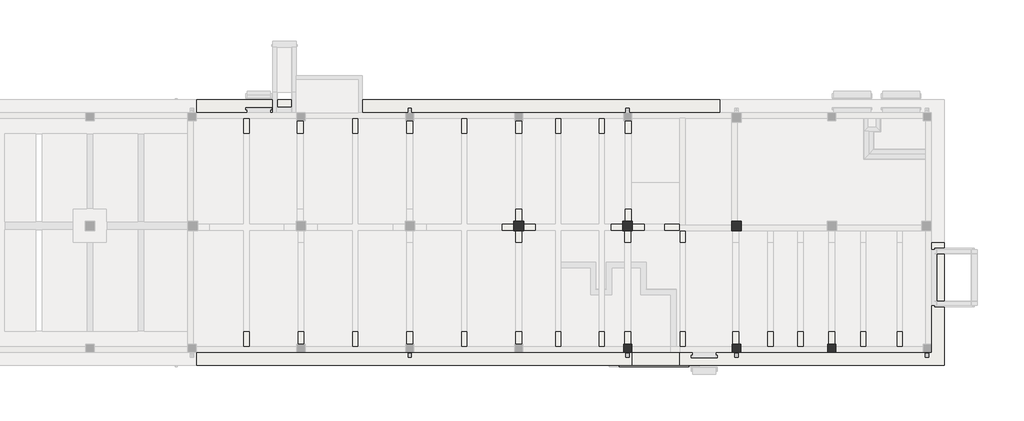
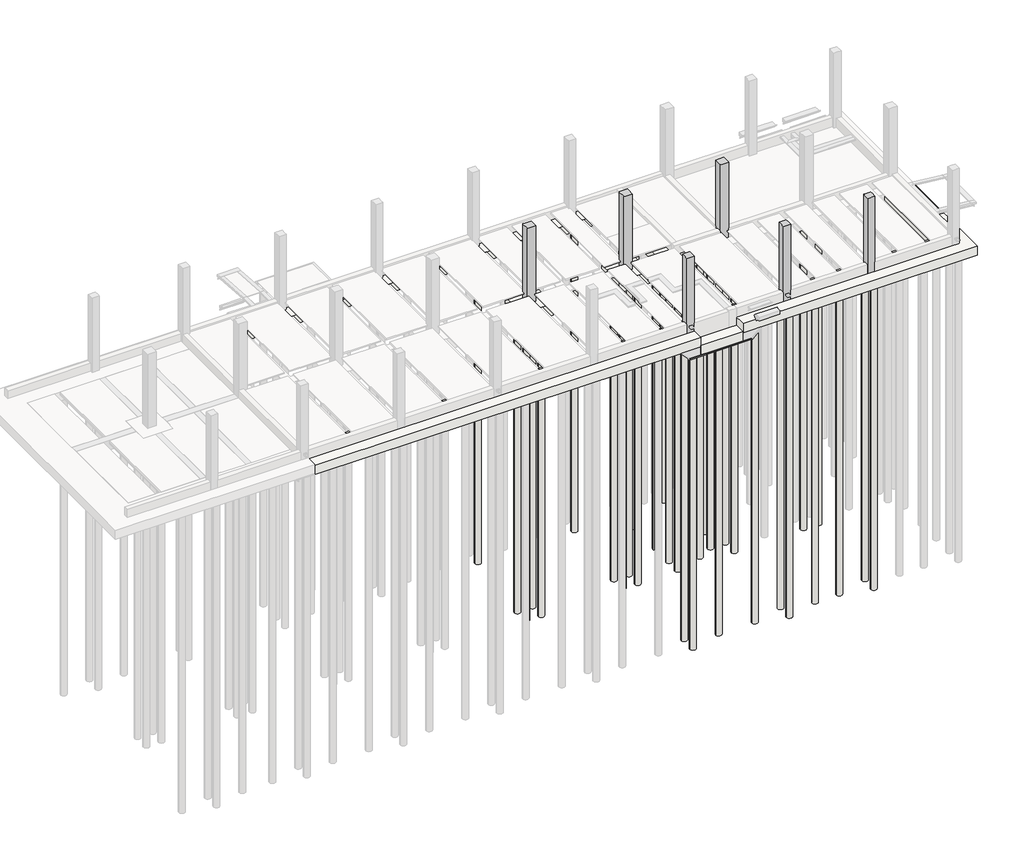
# One storey, part 5 of 7: 42 slabs, 6 columns.
"""IFC4 building model written with IfcOpenShell, lengths in millimetres."""

import ifcopenshell
import ifcopenshell.guid

model = None  # the IFC model being written
_history = None  # IfcOwnerHistory: only IFC2X3 demands one
_inside = {}  # id of a spatial element -> (the spatial element, [elements in it])
_under = {}  # id of a project, library or spatial element -> (it, [spatial elements below it])
_declared = {}  # id of a project -> (the project, [libraries it declares])
_typed = {}  # id of a type object -> (the type object, [elements of that type])
_made_of = {}  # id of a material, layer set ... -> (it, [elements and type objects made of it])


def new_model(schema):
    """Start an empty IFC model of exactly this schema.

    Asked for "IFC4X3", IfcOpenShell would pick the latest addendum, in which some entities
    have other attributes; the version numbers below select the first issue.
    IFC2X3 requires an IfcOwnerHistory on every rooted entity: one is made here for all.
    """
    global model, _history
    if schema == "IFC4X3":
        model = ifcopenshell.file(schema_version=(4, 3, 0, 0))
    else:
        model = ifcopenshell.file(schema=schema)
    _inside.clear()
    _under.clear()
    _declared.clear()
    _typed.clear()
    _made_of.clear()
    _history = None
    if model.schema == "IFC2X3":
        org = make("IfcOrganization", Name="unknown")
        user = make(
            "IfcPersonAndOrganization",
            ThePerson=make("IfcPerson", FamilyName="unknown"),
            TheOrganization=org,
        )
        app = make(
            "IfcApplication",
            ApplicationDeveloper=org,
            Version="unknown",
            ApplicationFullName="unknown",
            ApplicationIdentifier="unknown",
        )
        _history = make(
            "IfcOwnerHistory",
            OwningUser=user,
            OwningApplication=app,
            ChangeAction="ADDED",
            CreationDate=0,
        )
    return model


def make(cls, **values):
    """One entity of the class cls with the attributes given. An attribute that is None is left unset."""
    return model.create_entity(
        cls, **{name: value for name, value in values.items() if value is not None}
    )


def rooted(cls, **values):
    """An entity with a GlobalId (a new one), such as an element, a storey or a relation."""
    return make(cls, GlobalId=ifcopenshell.guid.new(), OwnerHistory=_history, **values)


def si_unit(unit_type, name, prefix=None):
    """IfcSIUnit, for example si_unit("LENGTHUNIT", "METRE", prefix="MILLI")."""
    return make("IfcSIUnit", UnitType=unit_type, Prefix=prefix, Name=name)


def assignment(units):
    """IfcUnitAssignment: the units of a project."""
    return None if units is None else make("IfcUnitAssignment", Units=units)


def point(xyz):
    """IfcCartesianPoint."""
    return None if xyz is None else make("IfcCartesianPoint", Coordinates=xyz)


def direction(xyz):
    """IfcDirection."""
    return None if xyz is None else make("IfcDirection", DirectionRatios=xyz)


def frame(location, z_axis=None, x_axis=None):
    """IfcAxis2Placement3D, a coordinate frame: its origin and axes. An axis left out is left unset."""
    return make(
        "IfcAxis2Placement3D",
        Location=point(location),
        Axis=direction(z_axis),
        RefDirection=direction(x_axis),
    )


def frame_2d(location, x_axis=None):
    """IfcAxis2Placement2D, a coordinate frame in the plane: its origin and x axis."""
    return make(
        "IfcAxis2Placement2D", Location=point(location), RefDirection=direction(x_axis)
    )


def origin():
    """The frame at (0, 0, 0) with its axes left unset."""
    return frame((0.0, 0.0, 0.0))


def place(relative_to, where):
    """IfcLocalPlacement: puts the frame where relative to a parent placement (None: the world)."""
    return make(
        "IfcLocalPlacement", PlacementRelTo=relative_to, RelativePlacement=where
    )


def context(
    kind, dimensions, precision=None, world=None, true_north=None, identifier=None
):
    """IfcGeometricRepresentationContext, for example the 3D "Model" context."""
    return make(
        "IfcGeometricRepresentationContext",
        ContextIdentifier=identifier,
        ContextType=kind,
        CoordinateSpaceDimension=dimensions,
        Precision=precision,
        WorldCoordinateSystem=world,
        TrueNorth=true_north,
    )


def project(units=None, contexts=None):
    """IfcProject with its units and contexts."""
    return rooted(
        "IfcProject",
        Name="project",
        RepresentationContexts=contexts,
        UnitsInContext=assignment(units),
    )


def spatial(cls, under=None, at=None, **own):
    """A site, building, storey or space (cls), placed at a placement, below another one or the project."""
    s = rooted(cls, ObjectPlacement=at, **own)
    if under is not None:
        _under.setdefault(under.id(), (under, []))[1].append(s)
    return s


def polyline(points):
    """IfcPolyline through the points."""
    return make("IfcPolyline", Points=[point(p) for p in points])


def circle_curve(where, radius):
    """IfcCircle in the frame where."""
    return make("IfcCircle", Position=where, Radius=radius)


def trimmed(basis, trim1, trim2, sense, master):
    """IfcTrimmedCurve: the piece of a basis curve between two trims."""
    return make(
        "IfcTrimmedCurve",
        BasisCurve=basis,
        Trim1=trim1,
        Trim2=trim2,
        SenseAgreement=sense,
        MasterRepresentation=master,
    )


def segment(curve, same_sense, transition):
    """IfcCompositeCurveSegment."""
    return make(
        "IfcCompositeCurveSegment",
        Transition=transition,
        SameSense=same_sense,
        ParentCurve=curve,
    )


def composite_curve(segments, self_intersect=None):
    """IfcCompositeCurve: segments joined end to end."""
    return make("IfcCompositeCurve", Segments=segments, SelfIntersect=self_intersect)


def outline(outer, holes=None, kind="AREA"):
    """IfcArbitraryClosedProfileDef: a profile drawn as a closed curve; with holes, ...WithVoids."""
    if holes is None:
        return make("IfcArbitraryClosedProfileDef", ProfileType=kind, OuterCurve=outer)
    return make(
        "IfcArbitraryProfileDefWithVoids",
        ProfileType=kind,
        OuterCurve=outer,
        InnerCurves=holes,
    )


def extrude(swept, where, along, depth):
    """IfcExtrudedAreaSolid: the profile swept, set in the frame where, extruded along a direction by depth."""
    return make(
        "IfcExtrudedAreaSolid",
        SweptArea=swept,
        Position=where,
        ExtrudedDirection=direction(along),
        Depth=depth,
    )


def faces_of(points, faces, orient=None, outer=None):
    """IfcFace entities. A face is a list of loops; a loop is a list of indices into points, from 0.

    orient and outer hold one flag for each loop. By default every Orientation is true, the
    first loop of a face is its IfcFaceOuterBound and the others are IfcFaceBound.
    """
    made = []
    for i, loops in enumerate(faces):
        bounds = []
        for j, loop in enumerate(loops):
            is_outer = j == 0 if outer is None else outer[i][j]
            bounds.append(
                make(
                    "IfcFaceOuterBound" if is_outer else "IfcFaceBound",
                    Bound=make("IfcPolyLoop", Polygon=[points[k] for k in loop]),
                    Orientation=True if orient is None else orient[i][j],
                )
            )
        made.append(make("IfcFace", Bounds=bounds))
    return made


def faceted_brep(points, faces, orient=None, outer=None, voids=None):
    """IfcFacetedBrep: a solid bounded by flat faces; with voids (closed shells), ...WithVoids."""
    shared = [point(p) for p in points]
    hull = make("IfcClosedShell", CfsFaces=faces_of(shared, faces, orient, outer))
    if voids is None:
        return make("IfcFacetedBrep", Outer=hull)
    return make(
        "IfcFacetedBrepWithVoids",
        Outer=hull,
        Voids=[
            make(cls, CfsFaces=faces_of(shared, fs, o, b)) for cls, fs, o, b in voids
        ],
    )


def shape(context_of_items, identifier, shape_type, items):
    """IfcShapeRepresentation: the items that make up one representation, for example the "Body"."""
    return make(
        "IfcShapeRepresentation",
        ContextOfItems=context_of_items,
        RepresentationIdentifier=identifier,
        RepresentationType=shape_type,
        Items=items,
    )


def made_of(thing, what):
    """Note that an element or type object is made of a material, layer set ...; save() writes the relation."""
    if what is not None:
        _made_of.setdefault(what.id(), (what, []))[1].append(thing)
    return thing


def element(
    cls,
    number,
    at=None,
    inside=None,
    cuts=None,
    type_object=None,
    material=None,
    context=None,
    identifier="Body",
    shape_type=None,
    held_by="IfcProductDefinitionShape",
    body=None,
    shapes=None,
    **own,
):
    """One element of the class cls, such as IfcWall. Its Tag is "e" and its number.

    at: its placement. inside: the storey or other place that contains it. cuts: it is an
    opening in that element (IfcRelVoidsElement). A single representation is given by context,
    identifier, shape_type and body (its items); several are given by shapes. held_by: the class
    of the entity that holds the representations. save() writes the other relations.
    """
    e = rooted(cls, Tag="e%d" % number, ObjectPlacement=at, **own)
    if body is not None:
        shapes = [shape(context, identifier, shape_type, body)]
    if shapes is not None:
        e.Representation = make(held_by, Representations=shapes)
    if inside is not None:
        _inside.setdefault(inside.id(), (inside, []))[1].append(e)
    if cuts is not None:
        rooted(
            "IfcRelVoidsElement", RelatingBuildingElement=cuts, RelatedOpeningElement=e
        )
    if type_object is not None:
        _typed.setdefault(type_object.id(), (type_object, []))[1].append(e)
    return made_of(e, material)


def aggregate(whole, parts):
    """IfcRelAggregates: a whole, such as a stair, and the parts it consists of."""
    return rooted("IfcRelAggregates", RelatingObject=whole, RelatedObjects=parts)


def save(model, path):
    """Write the relations noted so far, then the file.

    IfcRelAggregates (storeys below a building ...), IfcRelContainedInSpatialStructure (elements
    in a storey), IfcRelDefinesByType, IfcRelAssociatesMaterial and IfcRelDeclares: one each for
    every whole, place, type object, material and project.
    """
    for whole, parts in _under.values():
        aggregate(whole, parts)
    for where, things in _inside.values():
        rooted(
            "IfcRelContainedInSpatialStructure",
            RelatedElements=things,
            RelatingStructure=where,
        )
    for kind, things in _typed.values():
        rooted("IfcRelDefinesByType", RelatedObjects=things, RelatingType=kind)
    for what, things in _made_of.values():
        rooted("IfcRelAssociatesMaterial", RelatedObjects=things, RelatingMaterial=what)
    for by, libraries in _declared.values():
        rooted("IfcRelDeclares", RelatingContext=by, RelatedDefinitions=libraries)
    model.write(path)


model = new_model("IFC4")

# Units and contexts
model_context = context("Model", 3, world=origin())
ifc_project = project(units=[si_unit("LENGTHUNIT", "METRE", prefix="MILLI")], contexts=[model_context])

# Site, building, storey
site = spatial("IfcSite", under=ifc_project)
building = spatial("IfcBuilding", under=site)
storey = spatial("IfcBuildingStorey", under=building, Name="H.P.P", Elevation=4500.0)

# Columns
placement = place(None, origin())
element("IfcColumn", 1, ObjectType="RC_Column_Rectangular : H_SC_AR S15_RC Col-AG_700x700_C1", at=placement, inside=storey, context=model_context, shape_type="Brep", body=[
    faceted_brep([(39350.0000001, -7650.0, 4000.0), (39350.0000001, -8350.0, 4000.0), (39250.0000001, -8350.0, 4000.0), (38750.0000001, -8350.0, 4000.0), (38650.0000001, -8350.0, 4000.0), (38650.0000001, -7650.0, 4000.0), (38750.0, -7650.0, 4000.0), (39250.0, -7650.0, 4000.0), (39350.0000001, -7650.0, 4650.0), (39350.0000001, -7650.0, 4800.0), (39350.0000001, -7650.0, 10450.0), (39350.0000001, -7650.0, 10600.0), (39350.0000001, -7700.0, 10600.0), (39350.0000001, -8300.0, 10600.0), (39350.0000001, -8350.0, 10600.0), (39350.0000001, -8350.0, 10450.0), (39350.0000001, -8350.0, 4800.0), (39350.0000001, -8350.0, 4650.0), (39249.9999998, -8350.0, 10600.0), (38750.0000002, -8350.0, 10600.0), (38650.0000001, -8350.0, 10600.0), (38650.0000001, -8350.0, 10450.0), (38650.0000001, -8350.0, 4800.0), (38650.0000001, -8350.0, 4650.0), (38650.0000001, -8300.0, 10600.0), (38650.0000001, -7700.0, 10600.0), (38650.0000001, -7650.0, 10600.0), (38650.0000001, -7650.0, 10450.0), (38650.0000001, -7650.0, 4800.0), (38650.0000001, -7650.0, 4650.0), (38750.0000002, -7650.0, 10600.0), (39249.9999998, -7650.0, 10600.0)], [[[0, 1, 2, 3, 4, 5, 6, 7]], [[1, 0, 8, 9, 10, 11, 12, 13, 14, 15, 16, 17]], [[4, 3, 2, 1, 17, 16, 15, 14, 18, 19, 20, 21, 22, 23]], [[5, 4, 23, 22, 21, 20, 24, 25, 26, 27, 28, 29]], [[0, 7, 6, 5, 29, 28, 27, 26, 30, 31, 11, 10, 9, 8]], [[12, 11, 31, 30, 26, 25, 24, 20, 19, 18, 14, 13]]]),
])
element("IfcColumn", 2, ObjectType="RC_Column_Rectangular : H_SC_AR S15_RC Col-AG_700x700_C1", at=placement, inside=storey, context=model_context, shape_type="Brep", body=[
    faceted_brep([(47349.9999999, -7650.0, 4000.0), (47349.9999999, -8350.0, 4000.0), (47249.9999999, -8350.0, 4000.0), (46749.9999999, -8350.0, 4000.0), (46649.9999999, -8350.0, 4000.0), (46649.9999999, -7650.0, 4000.0), (46800.0, -7650.0, 4000.0), (47300.0, -7650.0, 4000.0), (47349.9999999, -7650.0, 4650.0), (47349.9999999, -7850.0, 4650.0), (47349.9999999, -7850.0, 4800.0), (47349.9999999, -7650.0, 4800.0), (47349.9999999, -7650.0, 10450.0), (47349.9999999, -7650.0, 10600.0), (47349.9999999, -7750.0, 10600.0), (47349.9999999, -8350.0, 10600.0), (47349.9999999, -8350.0, 10450.0), (47349.9999999, -8350.0, 4800.0), (47349.9999999, -8350.0, 4650.0), (47300.0, -8350.0, 10600.0), (46800.0, -8350.0, 10600.0), (46649.9999999, -8350.0, 10600.0), (46649.9999999, -8350.0, 10450.0), (46649.9999999, -8350.0, 4800.0), (46649.9999999, -8350.0, 4650.0), (46649.9999999, -8300.0, 10600.0), (46649.9999999, -7700.0, 10600.0), (46649.9999999, -7650.0, 10600.0), (46649.9999999, -7650.0, 10450.0), (46649.9999999, -7650.0, 4800.0), (46649.9999999, -7650.0, 4650.0), (46800.0, -7650.0, 10600.0), (47300.0, -7650.0, 10600.0), (47300.0, -7650.0, 4800.0), (47300.0, -7650.0, 4650.0), (47300.0, -7850.0, 4650.0), (47300.0, -7850.0, 4800.0)], [[[0, 1, 2, 3, 4, 5, 6, 7]], [[1, 0, 8, 9, 10, 11, 12, 13, 14, 15, 16, 17, 18]], [[4, 3, 2, 1, 18, 17, 16, 15, 19, 20, 21, 22, 23, 24]], [[5, 4, 24, 23, 22, 21, 25, 26, 27, 28, 29, 30]], [[0, 7, 6, 5, 30, 29, 28, 27, 31, 32, 13, 12, 11, 33, 34, 8]], [[14, 13, 32, 31, 27, 26, 25, 21, 20, 19, 15]], [[35, 9, 8, 34]], [[10, 36, 33, 11]], [[35, 36, 10, 9]], [[36, 35, 34, 33]]]),
])
element("IfcColumn", 3, ObjectType="RC_Column_Rectangular : H_SC_AR S15_RC Col-AG_700x700_C1", at=placement, inside=storey, context=model_context, shape_type="Brep", body=[
    faceted_brep([(55350.0, -7650.0, 4000.0), (55350.0, -7950.0, 4000.0), (55350.0, -8350.0, 4000.0), (54650.0, -8350.0, 4000.0), (54650.0, -7950.0, 4000.0), (54650.0, -7650.0, 4000.0), (55050.0, -7650.0, 4000.0), (55350.0, -7650.0, 10600.0), (55350.0, -8350.0, 10600.0), (55350.0, -8350.0, 10450.0), (55350.0, -8350.0, 9800.0), (55350.0, -8350.0, 4800.0), (55350.0, -8350.0, 4650.0), (55200.0, -8350.0, 10600.0), (54700.0, -8350.0, 10600.0), (54650.0, -8350.0, 10600.0), (54650.0, -8350.0, 10450.0), (54650.0, -8350.0, 9700.0), (54650.0, -8350.0, 4800.0), (54650.0, -8350.0, 4650.0), (54650.0, -7650.0, 10600.0), (54650.0, -7650.0, 9800.0), (54650.0, -7650.0, 4800.0)], [[[0, 1, 2, 3, 4, 5, 6]], [[2, 1, 0, 7, 8, 9, 10, 11, 12]], [[3, 2, 12, 11, 10, 9, 8, 13, 14, 15, 16, 17, 18, 19]], [[5, 4, 3, 19, 18, 17, 16, 15, 20, 21, 22]], [[0, 6, 5, 22, 21, 20, 7]], [[8, 7, 20, 15, 14, 13]]]),
])
element("IfcColumn", 4, ObjectType="RC_Column_Rectangular : H_SC_AR S15_RC Col-AG_600x600_C2", at=placement, inside=storey, context=model_context, shape_type="Brep", body=[
    faceted_brep([(62300.0, -16700.0, 4000.0), (62300.0, -16900.0, 4000.0), (62300.0, -17300.0, 4000.0), (61700.0, -17300.0, 4000.0), (61700.0, -16900.0, 4000.0), (61700.0, -16700.0, 4000.0), (62300.0, -16700.0, 4650.0), (62300.0, -16700.0, 4800.0), (62300.0, -16700.0, 10450.0), (62300.0, -16700.0, 10600.0), (62300.0, -16900.0, 10600.0), (62300.0, -17300.0, 10600.0), (62300.0, -17300.0, 9800.0), (62300.0, -17300.0, 4800.0), (61700.0, -17300.0, 10600.0), (61700.0, -17300.0, 9800.0), (61700.0, -17300.0, 4800.0), (61700.0, -16900.0, 10600.0), (61700.0, -16700.0, 10600.0), (61700.0, -16700.0, 10450.0), (61700.0, -16700.0, 4800.0), (61700.0, -16700.0, 4650.0), (61750.0, -16700.0, 10600.0), (62250.0, -16700.0, 10600.0)], [[[0, 1, 2, 3, 4, 5]], [[2, 1, 0, 6, 7, 8, 9, 10, 11, 12, 13]], [[3, 2, 13, 12, 11, 14, 15, 16]], [[5, 4, 3, 16, 15, 14, 17, 18, 19, 20, 21]], [[0, 5, 21, 20, 19, 18, 22, 23, 9, 8, 7, 6]], [[14, 11, 10, 9, 23, 22, 18, 17]]]),
])
element("IfcColumn", 5, ObjectType="RC_Column_Rectangular : H_SC_AR S15_RC Col-AG_600x600_C2", at=placement, inside=storey, context=model_context, shape_type="Brep", body=[
    faceted_brep([(55300.0, -16700.0, 4000.0), (55300.0, -16900.0, 4000.0), (55300.0, -17300.0, 4000.0), (54700.0, -17300.0, 4000.0), (54700.0, -16900.0, 4000.0), (54700.0, -16700.0, 4000.0), (55300.0, -16700.0, 4650.0), (55300.0, -16700.0, 4800.0), (55300.0, -16700.0, 10450.0), (55300.0, -16700.0, 10600.0), (55300.0, -16900.0, 10600.0), (55300.0, -17300.0, 10600.0), (55300.0, -17300.0, 9800.0), (55300.0, -17300.0, 4800.0), (54700.0, -17300.0, 10600.0), (54700.0, -17300.0, 9800.0), (54700.0, -17300.0, 4800.0), (54700.0, -16900.0, 10600.0), (54700.0, -16700.0, 10600.0), (54700.0, -16700.0, 10450.0), (54700.0, -16700.0, 9800.0), (54700.0, -16700.0, 4800.0), (54700.0, -16700.0, 4650.0), (55200.0, -16700.0, 10600.0)], [[[0, 1, 2, 3, 4, 5]], [[2, 1, 0, 6, 7, 8, 9, 10, 11, 12, 13]], [[3, 2, 13, 12, 11, 14, 15, 16]], [[5, 4, 3, 16, 15, 14, 17, 18, 19, 20, 21, 22]], [[0, 5, 22, 21, 20, 19, 18, 23, 9, 8, 7, 6]], [[14, 11, 10, 9, 23, 18, 17]]]),
])
element("IfcColumn", 6, ObjectType="RC_Column_Rectangular : H_SC_AR S15_RC Col-AG_600x600_C2", at=placement, inside=storey, context=model_context, shape_type="Brep", body=[
    faceted_brep([(46700.0, -16700.0, 4000.0), (47300.0, -16700.0, 4000.0), (47300.0, -17300.0, 4000.0), (46700.0, -17300.0, 4000.0), (46700.0, -16900.0, 4000.0), (46700.0, -16700.0, 4550.0), (46700.0, -16700.0, 4700.0), (46700.0, -16700.0, 10450.0), (46700.0, -16700.0, 10600.0), (46800.0, -16700.0, 10600.0), (47300.0, -16700.0, 10600.0), (47300.0, -16700.0, 10450.0), (47300.0, -16700.0, 4700.0), (47300.0, -16700.0, 4550.0), (47300.0, -16900.0, 10600.0), (47300.0, -17300.0, 10600.0), (47300.0, -17300.0, 9800.0), (47300.0, -17300.0, 4700.0), (46700.0, -17300.0, 10600.0), (46700.0, -17300.0, 9800.0), (46700.0, -17300.0, 4800.0), (46700.0, -16900.0, 10600.0)], [[[0, 1, 2, 3, 4]], [[1, 0, 5, 6, 7, 8, 9, 10, 11, 12, 13]], [[2, 1, 13, 12, 11, 10, 14, 15, 16, 17]], [[3, 2, 17, 16, 15, 18, 19, 20]], [[0, 4, 3, 20, 19, 18, 21, 8, 7, 6, 5]], [[18, 15, 14, 10, 9, 8, 21]]]),
])

# Slabs
element("IfcSlab", 7, ObjectType="H_SF_AR S18_MAT_T800_WF1", at=placement, inside=storey, context=model_context, shape_type="Brep", body=[
    faceted_brep([(50825.0, -18250.0000001, 3200.0), (50825.0, -15750.0000001, 3200.0), (52225.0, -15750.0000001, 3200.0), (67750.0000002, -15750.0000001, 3200.0), (67750.0000002, -9250.0, 3200.0), (70250.0, -9250.0, 3200.0), (70250.0, -18250.0000001, 3200.0), (52225.0, -18250.0000001, 3200.0), (50825.0, -18250.0000001, 4000.0), (70250.0, -18250.0000001, 4000.0), (70250.0, -9250.0, 4000.0), (67750.0000002, -9250.0, 4000.0), (67750.0000002, -15750.0000001, 4000.0), (50825.0, -15750.0000001, 4000.0), (50825.0, -16900.0, 4000.0), (50825.0, -18250.0000001, 3300.0), (50825.0, -15750.0000001, 3300.0)], [[[0, 1, 2, 3, 4, 5, 6, 7]], [[8, 9, 10, 11, 12, 13, 14]], [[6, 5, 10, 9]], [[0, 7, 6, 9, 8, 15]], [[3, 2, 1, 16, 13, 12]], [[4, 3, 12, 11]], [[1, 0, 15, 8, 14, 13, 16]], [[5, 4, 11, 10]]]),
    faceted_brep([(15299.9999999, -18250.0000001, 3200.0), (15299.9999999, -15750.0000001, 3200.0), (45675.0, -15750.0000001, 3200.0), (47300.0, -15750.0000001, 3200.0), (47300.0, -18250.0000001, 3200.0), (45675.0, -18250.0000001, 3200.0), (15299.9999999, -18250.0000001, 4000.0), (47300.0, -18250.0000001, 4000.0), (47300.0, -15750.0000001, 4000.0), (15299.9999999, -15750.0000001, 4000.0), (15299.9999999, -18250.0000001, 3300.0), (15299.9999999, -15750.0000001, 3300.0), (47300.0, -15750.0000001, 3300.0), (47300.0, -18250.0000001, 3300.0)], [[[0, 1, 2, 3, 4, 5]], [[6, 7, 8, 9]], [[1, 0, 10, 6, 9, 11]], [[3, 2, 1, 11, 9, 8, 12]], [[4, 3, 12, 8, 7, 13]], [[0, 5, 4, 13, 7, 6, 10]]]),
    faceted_brep([(53749.9998007, 1249.9999999, 3200.0), (53749.9998007, -1250.0000001, 3200.0), (52200.0000002, -1250.0000001, 3200.0), (52200.0000002, -6750.0000001, 3200.0), (53749.9998007, -6750.0000001, 3200.0), (53749.9998007, -9250.0, 3200.0), (49700.0000002, -9250.0, 3200.0), (49700.0000002, -1250.0000001, 3200.0), (15299.9999999, -1250.0000001, 3200.0), (15299.9999999, 1249.9999999, 3200.0), (53749.9998007, 1249.9999999, 4000.0), (15299.9999999, 1249.9999999, 4000.0), (15299.9999999, -1250.0000001, 4000.0), (49700.0000002, -1250.0000001, 4000.0), (49700.0000002, -9250.0, 4000.0), (53749.9998007, -9250.0, 4000.0), (53749.9998007, -6750.0000001, 4000.0), (52200.0000002, -6750.0000001, 4000.0), (52200.0000002, -1250.0000001, 4000.0), (53749.9998007, -1250.0000001, 4000.0), (15299.9999999, 1249.9999999, 3300.0), (15299.9999999, -1250.0000001, 3300.0)], [[[0, 1, 2, 3, 4, 5, 6, 7, 8, 9]], [[10, 11, 12, 13, 14, 15, 16, 17, 18, 19]], [[0, 9, 20, 11, 10]], [[6, 5, 15, 14]], [[7, 6, 14, 13]], [[8, 7, 13, 12, 21]], [[2, 1, 19, 18]], [[3, 2, 18, 17]], [[4, 3, 17, 16]], [[1, 0, 10, 19]], [[9, 8, 21, 12, 11, 20]], [[5, 4, 16, 15]]]),
])
element("IfcSlab", 8, ObjectType="H_SF_AR S18_MAT_T800_WF1", at=placement, inside=storey, context=model_context, shape_type="Brep", body=[
    faceted_brep([(50825.0, -15750.0000001, 2500.0), (50825.0, -18250.0000001, 2500.0), (47300.0, -18250.0000001, 2500.0), (47300.0, -15750.0000001, 2500.0), (50825.0, -18250.0000001, 3300.0), (50825.0, -15750.0000001, 3300.0), (47300.0, -15750.0000001, 3300.0), (47300.0, -18250.0000001, 3300.0), (50825.0, -15750.0000001, 3200.0), (50825.0, -18250.0000001, 3200.0), (47300.0, -18250.0000001, 3200.0), (47300.0, -15750.0000001, 3200.0)], [[[0, 1, 2, 3]], [[4, 5, 6, 7]], [[1, 0, 8, 5, 4, 9]], [[2, 1, 9, 4, 7, 10]], [[3, 2, 10, 7, 6, 11]], [[0, 3, 11, 6, 5, 8]]]),
])
element("IfcSlab", 9, ObjectType="H_SF_AR_S18_Lean_T50", at=placement, inside=storey, context=model_context, shape_type="SweptSolid", body=[
    extrude(outline(polyline([(51525.0, -15650.0), (51525.0, -18350.0000001), (46375.0, -18350.0000001), (46375.0, -15650.0), (51525.0, -15650.0)])), frame((0.0, 0.0, 2450.0), z_axis=(0.0, 0.0, 1.0), x_axis=(1.0, 0.0, 0.0)), (0.0, 0.0, 1.0), 50.0),
])
element("IfcSlab", 10, ObjectType="H_SF_AR_S18_Lean_T50", at=placement, inside=storey, context=model_context, shape_type="Brep", body=[
    faceted_brep([(50475.0, -16790.0, 4390.0), (47360.0, -16790.0, 4390.0), (47360.0, -10775.0, 4390.0), (48275.0, -10775.0, 4390.0), (48275.0, -12775.0, 4390.0), (50475.0, -12775.0, 4390.0), (47360.0, -16790.0, 4440.0), (50475.0, -16790.0, 4440.0), (50475.0, -12775.0, 4440.0), (48275.0, -12775.0, 4440.0), (48275.0, -10775.0, 4440.0), (47360.0, -10775.0, 4440.0)], [[[0, 1, 2, 3, 4, 5]], [[6, 7, 8, 9, 10, 11]], [[1, 0, 7, 6]], [[2, 1, 6, 11]], [[3, 2, 11, 10]], [[4, 3, 10, 9]], [[5, 4, 9, 8]], [[0, 5, 8, 7]]]),
    faceted_brep([(46640.0, -10775.0, 4390.0), (46640.0, -16790.0, 4390.0), (45435.0, -16790.0, 4390.0), (45435.0, -12775.0, 4390.0), (45504.2893219, -12775.0, 4390.0), (45525.0, -12775.0, 4390.0), (45525.0, -10775.0, 4390.0), (46640.0, -16790.0, 4440.0), (46640.0, -10775.0, 4440.0), (45525.0, -10775.0, 4440.0), (45525.0, -12775.0, 4440.0), (45454.2893219, -12775.0, 4440.0), (45435.0, -12775.0, 4440.0), (45435.0, -16790.0, 4440.0)], [[[0, 1, 2, 3, 4, 5, 6]], [[7, 8, 9, 10, 11, 12, 13]], [[1, 0, 8, 7]], [[2, 1, 7, 13]], [[3, 2, 13, 12]], [[3, 12, 11, 10, 5, 4]], [[6, 5, 10, 9]], [[0, 6, 9, 8]]]),
    faceted_brep([(44765.0, -12775.0, 4390.0), (44765.0, -16790.0, 4390.0), (42235.0, -16790.0, 4390.0), (42235.0, -10775.0, 4390.0), (44575.0, -10775.0, 4390.0), (44575.0, -12775.0, 4390.0), (44765.0, -16790.0, 4440.0), (44765.0, -12775.0, 4440.0), (44575.0, -12775.0, 4440.0), (44575.0, -10775.0, 4440.0), (42235.0, -10775.0, 4440.0), (42235.0, -16790.0, 4440.0)], [[[0, 1, 2, 3, 4, 5]], [[6, 7, 8, 9, 10, 11]], [[1, 0, 7, 6]], [[2, 1, 6, 11]], [[3, 2, 11, 10]], [[4, 3, 10, 9]], [[5, 4, 9, 8]], [[0, 5, 8, 7]]]),
    faceted_brep([(47410.0, -4825.0, 4390.0), (47410.0, -210.0, 4390.0), (50825.0, -210.0, 4390.0), (50825.0, -4825.0, 4390.0), (47410.0, -210.0, 4440.0), (47410.0, -4825.0, 4440.0), (50825.0, -4825.0, 4440.0), (50825.0, -210.0, 4440.0)], [[[0, 1, 2, 3]], [[4, 5, 6, 7]], [[1, 0, 5, 4]], [[2, 1, 4, 7]], [[3, 2, 7, 6]], [[0, 3, 6, 5]]]),
])
element("IfcSlab", 11, ObjectType="H_SF_AR_S18_Lean_T50", at=placement, inside=storey, context=model_context, shape_type="SweptSolid", body=[
    extrude(outline(polyline([(54650.0, -100.0), (54650.0, -7950.0), (51225.0, -7950.0), (51225.0, -100.0), (54650.0, -100.0)])), frame((0.0, 0.0, 4440.0), z_axis=(0.0, 0.0, 1.0), x_axis=(1.0, 0.0, 0.0)), (0.0, 0.0, 1.0), 50.0),
])
element("IfcSlab", 12, ObjectType="Foundation Rectangular (Non-Pile) : H_SF_AR S18_Ret Fdn_2500x2500xT1000_F1A", at=placement, inside=storey, context=model_context, shape_type="SweptSolid", body=[
    extrude(outline(polyline([(40250.0000001, -6750.0), (40250.0000001, -9250.0), (37750.0000001, -9250.0), (37750.0000001, -6750.0), (40250.0000001, -6750.0)])), frame((0.0, 0.0, 3000.0), z_axis=(0.0, 0.0, 1.0), x_axis=(1.0, 0.0, 0.0)), (0.0, 0.0, 1.0), 1000.0),
])
element("IfcSlab", 13, ObjectType="Foundation Rectangular (Non-Pile) : H_SF_AR S18_Ret Fdn_2500x2500xT1000_F1A", at=placement, inside=storey, context=model_context, shape_type="SweptSolid", body=[
    extrude(outline(polyline([(48249.9999999, -6750.0), (48249.9999999, -9250.0), (45749.9999999, -9250.0), (45749.9999999, -6750.0), (48249.9999999, -6750.0)])), frame((0.0, 0.0, 3000.0), z_axis=(0.0, 0.0, 1.0), x_axis=(1.0, 0.0, 0.0)), (0.0, 0.0, 1.0), 1000.0),
])
element("IfcSlab", 14, ObjectType="PILE : H_FL_AR S19_Pile_D500_L26.8", at=placement, inside=storey, context=model_context, shape_type="SweptSolid", body=[
    extrude(outline(composite_curve([segment(trimmed(circle_curve(frame_2d((39000.0, -625.0)), 250.0), [point((38750.0, -625.0))], [point((39250.0, -625.0))], False, "CARTESIAN"), True, "CONTINUOUS"), segment(trimmed(circle_curve(frame_2d((39000.0, -625.0)), 250.0), [point((39250.0, -625.0))], [point((38750.0, -625.0))], False, "CARTESIAN"), True, "CONTINUOUS")], self_intersect=False)), frame((0.0, 0.0, -23500.0), z_axis=(0.0, 0.0, 1.0), x_axis=(1.0, 0.0, 0.0)), (0.0, 0.0, 1.0), 26650.0),
])
element("IfcSlab", 15, ObjectType="PILE : H_FL_AR S19_Pile_D500_L26.8", at=placement, inside=storey, context=model_context, shape_type="SweptSolid", body=[
    extrude(outline(composite_curve([segment(trimmed(circle_curve(frame_2d((47000.0, -625.0000002)), 250.0), [point((46750.0, -625.0000002))], [point((47250.0, -625.0000002))], False, "CARTESIAN"), True, "CONTINUOUS"), segment(trimmed(circle_curve(frame_2d((47000.0, -625.0000002)), 250.0), [point((47250.0, -625.0000002))], [point((46750.0, -625.0000002))], False, "CARTESIAN"), True, "CONTINUOUS")], self_intersect=False)), frame((0.0, 0.0, -23500.0), z_axis=(0.0, 0.0, 1.0), x_axis=(1.0, 0.0, 0.0)), (0.0, 0.0, 1.0), 26650.0),
])
element("IfcSlab", 16, ObjectType="PILE : H_FL_AR S19_Pile_D500_L26.8", at=placement, inside=storey, context=model_context, shape_type="SweptSolid", body=[
    extrude(outline(composite_curve([segment(trimmed(circle_curve(frame_2d((50950.0000002, -625.0)), 250.0), [point((50700.0000002, -625.0))], [point((51200.0000002, -625.0))], False, "CARTESIAN"), True, "CONTINUOUS"), segment(trimmed(circle_curve(frame_2d((50950.0000002, -625.0)), 250.0), [point((51200.0000002, -625.0))], [point((50700.0000002, -625.0))], False, "CARTESIAN"), True, "CONTINUOUS")], self_intersect=False)), frame((0.0, 0.0, -23500.0), z_axis=(0.0, 0.0, 1.0), x_axis=(1.0, 0.0, 0.0)), (0.0, 0.0, 1.0), 26650.0),
])
element("IfcSlab", 17, ObjectType="PILE : H_FL_AR S19_Pile_D500_L26.8", at=placement, inside=storey, context=model_context, shape_type="SweptSolid", body=[
    extrude(outline(composite_curve([segment(trimmed(circle_curve(frame_2d((50950.0000002, -2500.0)), 250.0), [point((50700.0000002, -2500.0))], [point((51200.0000002, -2500.0))], False, "CARTESIAN"), True, "CONTINUOUS"), segment(trimmed(circle_curve(frame_2d((50950.0000002, -2500.0)), 250.0), [point((51200.0000002, -2500.0))], [point((50700.0000002, -2500.0))], False, "CARTESIAN"), True, "CONTINUOUS")], self_intersect=False)), frame((0.0, 0.0, -23500.0), z_axis=(0.0, 0.0, 1.0), x_axis=(1.0, 0.0, 0.0)), (0.0, 0.0, 1.0), 26650.0),
])
element("IfcSlab", 18, ObjectType="PILE : H_FL_AR S19_Pile_D500_L26.8", at=placement, inside=storey, context=model_context, shape_type="SweptSolid", body=[
    extrude(outline(composite_curve([segment(trimmed(circle_curve(frame_2d((50950.0000002, -5500.0)), 250.0), [point((50700.0000002, -5500.0))], [point((51200.0000002, -5500.0))], False, "CARTESIAN"), True, "CONTINUOUS"), segment(trimmed(circle_curve(frame_2d((50950.0000002, -5500.0)), 250.0), [point((51200.0000002, -5500.0))], [point((50700.0000002, -5500.0))], False, "CARTESIAN"), True, "CONTINUOUS")], self_intersect=False)), frame((0.0, 0.0, -23500.0), z_axis=(0.0, 0.0, 1.0), x_axis=(1.0, 0.0, 0.0)), (0.0, 0.0, 1.0), 26650.0),
])
element("IfcSlab", 19, ObjectType="PILE : H_FL_AR S19_Pile_D500_L26.8", at=placement, inside=storey, context=model_context, shape_type="SweptSolid", body=[
    extrude(outline(composite_curve([segment(trimmed(circle_curve(frame_2d((50950.0000002, -7375.0000222)), 250.0), [point((50700.0000002, -7375.0000222))], [point((51200.0000002, -7375.0000222))], False, "CARTESIAN"), True, "CONTINUOUS"), segment(trimmed(circle_curve(frame_2d((50950.0000002, -7375.0000222)), 250.0), [point((51200.0000002, -7375.0000222))], [point((50700.0000002, -7375.0000222))], False, "CARTESIAN"), True, "CONTINUOUS")], self_intersect=False)), frame((0.0, 0.0, -23500.0), z_axis=(0.0, 0.0, 1.0), x_axis=(1.0, 0.0, 0.0)), (0.0, 0.0, 1.0), 26650.0),
])
element("IfcSlab", 20, ObjectType="PILE : H_FL_AR S19_Pile_D500_L26.8", at=placement, inside=storey, context=model_context, shape_type="SweptSolid", body=[
    extrude(outline(composite_curve([segment(trimmed(circle_curve(frame_2d((50950.0000002, -8625.0000222)), 250.0), [point((50700.0000002, -8625.0000222))], [point((51200.0000002, -8625.0000222))], False, "CARTESIAN"), True, "CONTINUOUS"), segment(trimmed(circle_curve(frame_2d((50950.0000002, -8625.0000222)), 250.0), [point((51200.0000002, -8625.0000222))], [point((50700.0000002, -8625.0000222))], False, "CARTESIAN"), True, "CONTINUOUS")], self_intersect=False)), frame((0.0, 0.0, -23500.0), z_axis=(0.0, 0.0, 1.0), x_axis=(1.0, 0.0, 0.0)), (0.0, 0.0, 1.0), 26650.0),
])
element("IfcSlab", 21, ObjectType="PILE : H_FL_AR S19_Pile_D500_L26.8", at=placement, inside=storey, context=model_context, shape_type="SweptSolid", body=[
    extrude(outline(composite_curve([segment(trimmed(circle_curve(frame_2d((53125.0, -8000.0)), 250.0), [point((52875.0, -8000.0))], [point((53375.0, -8000.0))], False, "CARTESIAN"), True, "CONTINUOUS"), segment(trimmed(circle_curve(frame_2d((53125.0, -8000.0)), 250.0), [point((53375.0, -8000.0))], [point((52875.0, -8000.0))], False, "CARTESIAN"), True, "CONTINUOUS")], self_intersect=False)), frame((0.0, 0.0, -23500.0), z_axis=(0.0, 0.0, 1.0), x_axis=(1.0, 0.0, 0.0)), (0.0, 0.0, 1.0), 26650.0),
])
element("IfcSlab", 22, ObjectType="PILE : H_FL_AR S19_Pile_D500_L26.6", at=placement, inside=storey, context=model_context, shape_type="SweptSolid", body=[
    extrude(outline(composite_curve([segment(trimmed(circle_curve(frame_2d((38375.0000004, -7374.9999999)), 250.0), [point((38125.0000004, -7374.9999999))], [point((38625.0000004, -7374.9999999))], False, "CARTESIAN"), True, "CONTINUOUS"), segment(trimmed(circle_curve(frame_2d((38375.0000004, -7374.9999999)), 250.0), [point((38625.0000004, -7374.9999999))], [point((38125.0000004, -7374.9999999))], False, "CARTESIAN"), True, "CONTINUOUS")], self_intersect=False)), frame((0.0, 0.0, -23500.0), z_axis=(0.0, 0.0, 1.0), x_axis=(1.0, 0.0, 0.0)), (0.0, 0.0, 1.0), 26450.0),
])
element("IfcSlab", 23, ObjectType="PILE : H_FL_AR S19_Pile_D500_L26.6", at=placement, inside=storey, context=model_context, shape_type="SweptSolid", body=[
    extrude(outline(composite_curve([segment(trimmed(circle_curve(frame_2d((39625.0000004, -7374.9999999)), 250.0), [point((39375.0000004, -7374.9999999))], [point((39875.0000004, -7374.9999999))], False, "CARTESIAN"), True, "CONTINUOUS"), segment(trimmed(circle_curve(frame_2d((39625.0000004, -7374.9999999)), 250.0), [point((39875.0000004, -7374.9999999))], [point((39375.0000004, -7374.9999999))], False, "CARTESIAN"), True, "CONTINUOUS")], self_intersect=False)), frame((0.0, 0.0, -23500.0), z_axis=(0.0, 0.0, 1.0), x_axis=(1.0, 0.0, 0.0)), (0.0, 0.0, 1.0), 26450.0),
])
element("IfcSlab", 24, ObjectType="PILE : H_FL_AR S19_Pile_D500_L26.6", at=placement, inside=storey, context=model_context, shape_type="SweptSolid", body=[
    extrude(outline(composite_curve([segment(trimmed(circle_curve(frame_2d((38375.0000004, -8624.9999999)), 250.0), [point((38125.0000004, -8624.9999999))], [point((38625.0000004, -8624.9999999))], False, "CARTESIAN"), True, "CONTINUOUS"), segment(trimmed(circle_curve(frame_2d((38375.0000004, -8624.9999999)), 250.0), [point((38625.0000004, -8624.9999999))], [point((38125.0000004, -8624.9999999))], False, "CARTESIAN"), True, "CONTINUOUS")], self_intersect=False)), frame((0.0, 0.0, -23500.0), z_axis=(0.0, 0.0, 1.0), x_axis=(1.0, 0.0, 0.0)), (0.0, 0.0, 1.0), 26450.0),
])
element("IfcSlab", 25, ObjectType="PILE : H_FL_AR S19_Pile_D500_L26.6", at=placement, inside=storey, context=model_context, shape_type="SweptSolid", body=[
    extrude(outline(composite_curve([segment(trimmed(circle_curve(frame_2d((39625.0000004, -8624.9999999)), 250.0), [point((39375.0000004, -8624.9999999))], [point((39875.0000004, -8624.9999999))], False, "CARTESIAN"), True, "CONTINUOUS"), segment(trimmed(circle_curve(frame_2d((39625.0000004, -8624.9999999)), 250.0), [point((39875.0000004, -8624.9999999))], [point((39375.0000004, -8624.9999999))], False, "CARTESIAN"), True, "CONTINUOUS")], self_intersect=False)), frame((0.0, 0.0, -23500.0), z_axis=(0.0, 0.0, 1.0), x_axis=(1.0, 0.0, 0.0)), (0.0, 0.0, 1.0), 26450.0),
])
element("IfcSlab", 26, ObjectType="PILE : H_FL_AR S19_Pile_D500_L26.6", at=placement, inside=storey, context=model_context, shape_type="SweptSolid", body=[
    extrude(outline(composite_curve([segment(trimmed(circle_curve(frame_2d((46375.0000004, -7374.9999999)), 250.0), [point((46125.0000004, -7374.9999999))], [point((46625.0000004, -7374.9999999))], False, "CARTESIAN"), True, "CONTINUOUS"), segment(trimmed(circle_curve(frame_2d((46375.0000004, -7374.9999999)), 250.0), [point((46625.0000004, -7374.9999999))], [point((46125.0000004, -7374.9999999))], False, "CARTESIAN"), True, "CONTINUOUS")], self_intersect=False)), frame((0.0, 0.0, -23500.0), z_axis=(0.0, 0.0, 1.0), x_axis=(1.0, 0.0, 0.0)), (0.0, 0.0, 1.0), 26450.0),
])
element("IfcSlab", 27, ObjectType="PILE : H_FL_AR S19_Pile_D500_L26.6", at=placement, inside=storey, context=model_context, shape_type="SweptSolid", body=[
    extrude(outline(composite_curve([segment(trimmed(circle_curve(frame_2d((47625.0000004, -7374.9999999)), 250.0), [point((47375.0000004, -7374.9999999))], [point((47875.0000004, -7374.9999999))], False, "CARTESIAN"), True, "CONTINUOUS"), segment(trimmed(circle_curve(frame_2d((47625.0000004, -7374.9999999)), 250.0), [point((47875.0000004, -7374.9999999))], [point((47375.0000004, -7374.9999999))], False, "CARTESIAN"), True, "CONTINUOUS")], self_intersect=False)), frame((0.0, 0.0, -23500.0), z_axis=(0.0, 0.0, 1.0), x_axis=(1.0, 0.0, 0.0)), (0.0, 0.0, 1.0), 26450.0),
])
element("IfcSlab", 28, ObjectType="PILE : H_FL_AR S19_Pile_D500_L26.6", at=placement, inside=storey, context=model_context, shape_type="SweptSolid", body=[
    extrude(outline(composite_curve([segment(trimmed(circle_curve(frame_2d((46375.0000004, -8624.9999999)), 250.0), [point((46125.0000004, -8624.9999999))], [point((46625.0000004, -8624.9999999))], False, "CARTESIAN"), True, "CONTINUOUS"), segment(trimmed(circle_curve(frame_2d((46375.0000004, -8624.9999999)), 250.0), [point((46625.0000004, -8624.9999999))], [point((46125.0000004, -8624.9999999))], False, "CARTESIAN"), True, "CONTINUOUS")], self_intersect=False)), frame((0.0, 0.0, -23500.0), z_axis=(0.0, 0.0, 1.0), x_axis=(1.0, 0.0, 0.0)), (0.0, 0.0, 1.0), 26450.0),
])
element("IfcSlab", 29, ObjectType="PILE : H_FL_AR S19_Pile_D500_L26.6", at=placement, inside=storey, context=model_context, shape_type="SweptSolid", body=[
    extrude(outline(composite_curve([segment(trimmed(circle_curve(frame_2d((47625.0000004, -8624.9999999)), 250.0), [point((47375.0000004, -8624.9999999))], [point((47875.0000004, -8624.9999999))], False, "CARTESIAN"), True, "CONTINUOUS"), segment(trimmed(circle_curve(frame_2d((47625.0000004, -8624.9999999)), 250.0), [point((47875.0000004, -8624.9999999))], [point((47375.0000004, -8624.9999999))], False, "CARTESIAN"), True, "CONTINUOUS")], self_intersect=False)), frame((0.0, 0.0, -23500.0), z_axis=(0.0, 0.0, 1.0), x_axis=(1.0, 0.0, 0.0)), (0.0, 0.0, 1.0), 26450.0),
])
element("IfcSlab", 30, ObjectType="PILE : H_FL_AR S19_Pile_D500_L26.1", at=placement, inside=storey, context=model_context, shape_type="SweptSolid", body=[
    extrude(outline(composite_curve([segment(trimmed(circle_curve(frame_2d((47000.0, -16375.0000002)), 250.0), [point((47250.0, -16375.0000002))], [point((46750.0, -16375.0000002))], False, "CARTESIAN"), True, "CONTINUOUS"), segment(trimmed(circle_curve(frame_2d((47000.0, -16375.0000002)), 250.0), [point((46750.0, -16375.0000002))], [point((47250.0, -16375.0000002))], False, "CARTESIAN"), True, "CONTINUOUS")], self_intersect=False)), frame((0.0, 0.0, 2500.0), z_axis=(0.0, 0.0, 1.0), x_axis=(1.0, 0.0, 0.0)), (0.0, 0.0, 1.0), 100.0),
    extrude(outline(composite_curve([segment(trimmed(circle_curve(frame_2d((47000.0, -16375.0000002)), 250.0), [point((46750.0, -16375.0000002))], [point((47250.0, -16375.0000002))], False, "CARTESIAN"), True, "CONTINUOUS"), segment(trimmed(circle_curve(frame_2d((47000.0, -16375.0000002)), 250.0), [point((47250.0, -16375.0000002))], [point((46750.0, -16375.0000002))], False, "CARTESIAN"), True, "CONTINUOUS")], self_intersect=False)), frame((0.0, 0.0, -23500.0), z_axis=(0.0, 0.0, 1.0), x_axis=(1.0, 0.0, 0.0)), (0.0, 0.0, 1.0), 25950.0),
])
element("IfcSlab", 31, ObjectType="PILE : H_FL_AR S19_Pile_D500_L26.1", at=placement, inside=storey, context=model_context, shape_type="SweptSolid", body=[
    extrude(outline(composite_curve([segment(trimmed(circle_curve(frame_2d((47000.0, -17624.9999997)), 250.0), [point((47250.0, -17624.9999997))], [point((46750.0, -17624.9999997))], False, "CARTESIAN"), True, "CONTINUOUS"), segment(trimmed(circle_curve(frame_2d((47000.0, -17624.9999997)), 250.0), [point((46750.0, -17624.9999997))], [point((47250.0, -17624.9999997))], False, "CARTESIAN"), True, "CONTINUOUS")], self_intersect=False)), frame((0.0, 0.0, 2500.0), z_axis=(0.0, 0.0, 1.0), x_axis=(1.0, 0.0, 0.0)), (0.0, 0.0, 1.0), 100.0),
    extrude(outline(composite_curve([segment(trimmed(circle_curve(frame_2d((47000.0, -17624.9999997)), 250.0), [point((46750.0, -17624.9999997))], [point((47250.0, -17624.9999997))], False, "CARTESIAN"), True, "CONTINUOUS"), segment(trimmed(circle_curve(frame_2d((47000.0, -17624.9999997)), 250.0), [point((47250.0, -17624.9999997))], [point((46750.0, -17624.9999997))], False, "CARTESIAN"), True, "CONTINUOUS")], self_intersect=False)), frame((0.0, 0.0, -23500.0), z_axis=(0.0, 0.0, 1.0), x_axis=(1.0, 0.0, 0.0)), (0.0, 0.0, 1.0), 25950.0),
])
element("IfcSlab", 32, ObjectType="PILE : H_FL_AR S19_Pile_D500_L26.1", at=placement, inside=storey, context=model_context, shape_type="SweptSolid", body=[
    extrude(outline(composite_curve([segment(trimmed(circle_curve(frame_2d((49500.0000012, -17000.0)), 250.0), [point((49250.0000012, -17000.0))], [point((49750.0000012, -17000.0))], False, "CARTESIAN"), True, "CONTINUOUS"), segment(trimmed(circle_curve(frame_2d((49500.0000012, -17000.0)), 250.0), [point((49750.0000012, -17000.0))], [point((49250.0000012, -17000.0))], False, "CARTESIAN"), True, "CONTINUOUS")], self_intersect=False)), frame((0.0, 0.0, -23500.0), z_axis=(0.0, 0.0, 1.0), x_axis=(1.0, 0.0, 0.0)), (0.0, 0.0, 1.0), 25950.0),
])
element("IfcSlab", 33, ObjectType="PILE : H_FL_AR S19_Pile_D500_L26.8", at=placement, inside=storey, context=model_context, shape_type="SweptSolid", body=[
    extrude(outline(composite_curve([segment(trimmed(circle_curve(frame_2d((52500.0000003, -17000.0)), 250.0), [point((52250.0000003, -17000.0))], [point((52750.0000003, -17000.0))], False, "CARTESIAN"), True, "CONTINUOUS"), segment(trimmed(circle_curve(frame_2d((52500.0000003, -17000.0)), 250.0), [point((52750.0000003, -17000.0))], [point((52250.0000003, -17000.0))], False, "CARTESIAN"), True, "CONTINUOUS")], self_intersect=False)), frame((0.0, 0.0, -23500.0), z_axis=(0.0, 0.0, 1.0), x_axis=(1.0, 0.0, 0.0)), (0.0, 0.0, 1.0), 26650.0),
])
element("IfcSlab", 34, ObjectType="PILE : H_FL_AR S19_Pile_D500_L26.8", at=placement, inside=storey, context=model_context, shape_type="SweptSolid", body=[
    extrude(outline(composite_curve([segment(trimmed(circle_curve(frame_2d((55000.0, -16375.0000004)), 250.0), [point((54750.0, -16375.0000004))], [point((55250.0, -16375.0000004))], False, "CARTESIAN"), True, "CONTINUOUS"), segment(trimmed(circle_curve(frame_2d((55000.0, -16375.0000004)), 250.0), [point((55250.0, -16375.0000004))], [point((54750.0, -16375.0000004))], False, "CARTESIAN"), True, "CONTINUOUS")], self_intersect=False)), frame((0.0, 0.0, -23500.0), z_axis=(0.0, 0.0, 1.0), x_axis=(1.0, 0.0, 0.0)), (0.0, 0.0, 1.0), 26650.0),
])
element("IfcSlab", 35, ObjectType="PILE : H_FL_AR S19_Pile_D500_L26.8", at=placement, inside=storey, context=model_context, shape_type="SweptSolid", body=[
    extrude(outline(composite_curve([segment(trimmed(circle_curve(frame_2d((55000.0, -17625.0)), 250.0), [point((54750.0, -17625.0))], [point((55250.0, -17625.0))], False, "CARTESIAN"), True, "CONTINUOUS"), segment(trimmed(circle_curve(frame_2d((55000.0, -17625.0)), 250.0), [point((55250.0, -17625.0))], [point((54750.0, -17625.0))], False, "CARTESIAN"), True, "CONTINUOUS")], self_intersect=False)), frame((0.0, 0.0, -23500.0), z_axis=(0.0, 0.0, 1.0), x_axis=(1.0, 0.0, 0.0)), (0.0, 0.0, 1.0), 26650.0),
])
element("IfcSlab", 36, ObjectType="PILE : H_FL_AR S19_Pile_D500_L26.8", at=placement, inside=storey, context=model_context, shape_type="SweptSolid", body=[
    extrude(outline(composite_curve([segment(trimmed(circle_curve(frame_2d((57499.9999998, -17000.0)), 250.0), [point((57249.9999998, -17000.0))], [point((57749.9999998, -17000.0))], False, "CARTESIAN"), True, "CONTINUOUS"), segment(trimmed(circle_curve(frame_2d((57499.9999998, -17000.0)), 250.0), [point((57749.9999998, -17000.0))], [point((57249.9999998, -17000.0))], False, "CARTESIAN"), True, "CONTINUOUS")], self_intersect=False)), frame((0.0, 0.0, -23500.0), z_axis=(0.0, 0.0, 1.0), x_axis=(1.0, 0.0, 0.0)), (0.0, 0.0, 1.0), 26650.0),
])
element("IfcSlab", 37, ObjectType="PILE : H_FL_AR S19_Pile_D500_L26.8", at=placement, inside=storey, context=model_context, shape_type="SweptSolid", body=[
    extrude(outline(composite_curve([segment(trimmed(circle_curve(frame_2d((59500.0, -17000.0)), 250.0), [point((59250.0, -17000.0))], [point((59750.0, -17000.0))], False, "CARTESIAN"), True, "CONTINUOUS"), segment(trimmed(circle_curve(frame_2d((59500.0, -17000.0)), 250.0), [point((59750.0, -17000.0))], [point((59250.0, -17000.0))], False, "CARTESIAN"), True, "CONTINUOUS")], self_intersect=False)), frame((0.0, 0.0, -23500.0), z_axis=(0.0, 0.0, 1.0), x_axis=(1.0, 0.0, 0.0)), (0.0, 0.0, 1.0), 26650.0),
])
element("IfcSlab", 38, ObjectType="PILE : H_FL_AR S19_Pile_D500_L26.8", at=placement, inside=storey, context=model_context, shape_type="SweptSolid", body=[
    extrude(outline(composite_curve([segment(trimmed(circle_curve(frame_2d((62000.0, -16375.0)), 250.0), [point((61750.0, -16375.0))], [point((62250.0, -16375.0))], False, "CARTESIAN"), True, "CONTINUOUS"), segment(trimmed(circle_curve(frame_2d((62000.0, -16375.0)), 250.0), [point((62250.0, -16375.0))], [point((61750.0, -16375.0))], False, "CARTESIAN"), True, "CONTINUOUS")], self_intersect=False)), frame((0.0, 0.0, -23500.0), z_axis=(0.0, 0.0, 1.0), x_axis=(1.0, 0.0, 0.0)), (0.0, 0.0, 1.0), 26650.0),
])
element("IfcSlab", 39, ObjectType="PILE : H_FL_AR S19_Pile_D500_L26.8", at=placement, inside=storey, context=model_context, shape_type="SweptSolid", body=[
    extrude(outline(composite_curve([segment(trimmed(circle_curve(frame_2d((62000.0, -17624.9999996)), 250.0), [point((61750.0, -17624.9999996))], [point((62250.0, -17624.9999996))], False, "CARTESIAN"), True, "CONTINUOUS"), segment(trimmed(circle_curve(frame_2d((62000.0, -17624.9999996)), 250.0), [point((62250.0, -17624.9999996))], [point((61750.0, -17624.9999996))], False, "CARTESIAN"), True, "CONTINUOUS")], self_intersect=False)), frame((0.0, 0.0, -23500.0), z_axis=(0.0, 0.0, 1.0), x_axis=(1.0, 0.0, 0.0)), (0.0, 0.0, 1.0), 26650.0),
])
element("IfcSlab", 40, ObjectType="PILE : H_FL_AR S19_Pile_D500_L26.8", at=placement, inside=storey, context=model_context, shape_type="SweptSolid", body=[
    extrude(outline(composite_curve([segment(trimmed(circle_curve(frame_2d((62625.0000001, -8625.0)), 250.0), [point((62375.0000001, -8625.0))], [point((62875.0000001, -8625.0))], False, "CARTESIAN"), True, "CONTINUOUS"), segment(trimmed(circle_curve(frame_2d((62625.0000001, -8625.0)), 250.0), [point((62875.0000001, -8625.0))], [point((62375.0000001, -8625.0))], False, "CARTESIAN"), True, "CONTINUOUS")], self_intersect=False)), frame((0.0, 0.0, -23500.0), z_axis=(0.0, 0.0, 1.0), x_axis=(1.0, 0.0, 0.0)), (0.0, 0.0, 1.0), 26650.0),
])
element("IfcSlab", 41, ObjectType="PILE : H_FL_AR S19_Pile_D500_L26.8", at=placement, inside=storey, context=model_context, shape_type="SweptSolid", body=[
    extrude(outline(composite_curve([segment(trimmed(circle_curve(frame_2d((61375.0000001, -8625.0)), 250.0), [point((61125.0000001, -8625.0))], [point((61625.0000001, -8625.0))], False, "CARTESIAN"), True, "CONTINUOUS"), segment(trimmed(circle_curve(frame_2d((61375.0000001, -8625.0)), 250.0), [point((61625.0000001, -8625.0))], [point((61125.0000001, -8625.0))], False, "CARTESIAN"), True, "CONTINUOUS")], self_intersect=False)), frame((0.0, 0.0, -23500.0), z_axis=(0.0, 0.0, 1.0), x_axis=(1.0, 0.0, 0.0)), (0.0, 0.0, 1.0), 26650.0),
])
element("IfcSlab", 42, ObjectType="PILE : H_FL_AR S19_Pile_D500_L26.8", at=placement, inside=storey, context=model_context, shape_type="SweptSolid", body=[
    extrude(outline(composite_curve([segment(trimmed(circle_curve(frame_2d((55625.0, -8625.0)), 250.0), [point((55375.0, -8625.0))], [point((55875.0, -8625.0))], False, "CARTESIAN"), True, "CONTINUOUS"), segment(trimmed(circle_curve(frame_2d((55625.0, -8625.0)), 250.0), [point((55875.0, -8625.0))], [point((55375.0, -8625.0))], False, "CARTESIAN"), True, "CONTINUOUS")], self_intersect=False)), frame((0.0, 0.0, -23500.0), z_axis=(0.0, 0.0, 1.0), x_axis=(1.0, 0.0, 0.0)), (0.0, 0.0, 1.0), 26650.0),
])
element("IfcSlab", 43, ObjectType="PILE : H_FL_AR S19_Pile_D500_L26.8", at=placement, inside=storey, context=model_context, shape_type="SweptSolid", body=[
    extrude(outline(composite_curve([segment(trimmed(circle_curve(frame_2d((55625.0, -7375.0)), 250.0), [point((55375.0, -7375.0))], [point((55875.0, -7375.0))], False, "CARTESIAN"), True, "CONTINUOUS"), segment(trimmed(circle_curve(frame_2d((55625.0, -7375.0)), 250.0), [point((55875.0, -7375.0))], [point((55375.0, -7375.0))], False, "CARTESIAN"), True, "CONTINUOUS")], self_intersect=False)), frame((0.0, 0.0, -23500.0), z_axis=(0.0, 0.0, 1.0), x_axis=(1.0, 0.0, 0.0)), (0.0, 0.0, 1.0), 26650.0),
])
element("IfcSlab", 44, ObjectType="PILE : H_FL_AR S19_Pile_D500_L26.8", at=placement, inside=storey, context=model_context, shape_type="SweptSolid", body=[
    extrude(outline(composite_curve([segment(trimmed(circle_curve(frame_2d((54375.0, -7375.0)), 250.0), [point((54125.0, -7375.0))], [point((54625.0, -7375.0))], False, "CARTESIAN"), True, "CONTINUOUS"), segment(trimmed(circle_curve(frame_2d((54375.0, -7375.0)), 250.0), [point((54625.0, -7375.0))], [point((54125.0, -7375.0))], False, "CARTESIAN"), True, "CONTINUOUS")], self_intersect=False)), frame((0.0, 0.0, -23500.0), z_axis=(0.0, 0.0, 1.0), x_axis=(1.0, 0.0, 0.0)), (0.0, 0.0, 1.0), 26650.0),
])
element("IfcSlab", 45, ObjectType="PILE : H_FL_AR S19_Pile_D500_L26.8", at=placement, inside=storey, context=model_context, shape_type="SweptSolid", body=[
    extrude(outline(composite_curve([segment(trimmed(circle_curve(frame_2d((54375.0, -8625.0)), 250.0), [point((54125.0, -8625.0))], [point((54625.0, -8625.0))], False, "CARTESIAN"), True, "CONTINUOUS"), segment(trimmed(circle_curve(frame_2d((54375.0, -8625.0)), 250.0), [point((54625.0, -8625.0))], [point((54125.0, -8625.0))], False, "CARTESIAN"), True, "CONTINUOUS")], self_intersect=False)), frame((0.0, 0.0, -23500.0), z_axis=(0.0, 0.0, 1.0), x_axis=(1.0, 0.0, 0.0)), (0.0, 0.0, 1.0), 26650.0),
])
element("IfcSlab", 46, ObjectType="PILE : H_FL_AR S19_Pile_D500_L26.8", at=placement, inside=storey, context=model_context, shape_type="SweptSolid", body=[
    extrude(outline(composite_curve([segment(trimmed(circle_curve(frame_2d((55000.0, -5499.9999996)), 250.0), [point((54750.0, -5499.9999996))], [point((55250.0, -5499.9999996))], False, "CARTESIAN"), True, "CONTINUOUS"), segment(trimmed(circle_curve(frame_2d((55000.0, -5499.9999996)), 250.0), [point((55250.0, -5499.9999996))], [point((54750.0, -5499.9999996))], False, "CARTESIAN"), True, "CONTINUOUS")], self_intersect=False)), frame((0.0, 0.0, -23500.0), z_axis=(0.0, 0.0, 1.0), x_axis=(1.0, 0.0, 0.0)), (0.0, 0.0, 1.0), 26650.0),
])
element("IfcSlab", 47, ObjectType="PILE : H_FL_AR S19_Pile_D500_L26.8", at=placement, inside=storey, context=model_context, shape_type="SweptSolid", body=[
    extrude(outline(composite_curve([segment(trimmed(circle_curve(frame_2d((55000.0, -2500.0000004)), 250.0), [point((54750.0, -2500.0000004))], [point((55250.0, -2500.0000004))], False, "CARTESIAN"), True, "CONTINUOUS"), segment(trimmed(circle_curve(frame_2d((55000.0, -2500.0000004)), 250.0), [point((55250.0, -2500.0000004))], [point((54750.0, -2500.0000004))], False, "CARTESIAN"), True, "CONTINUOUS")], self_intersect=False)), frame((0.0, 0.0, -23500.0), z_axis=(0.0, 0.0, 1.0), x_axis=(1.0, 0.0, 0.0)), (0.0, 0.0, 1.0), 26650.0),
])
element("IfcSlab", 48, ObjectType="PILE : H_FL_AR S19_Pile_D500_L26.8", at=placement, inside=storey, context=model_context, shape_type="SweptSolid", body=[
    extrude(outline(composite_curve([segment(trimmed(circle_curve(frame_2d((54375.0, -625.0)), 250.0), [point((54125.0, -625.0))], [point((54625.0, -625.0))], False, "CARTESIAN"), True, "CONTINUOUS"), segment(trimmed(circle_curve(frame_2d((54375.0, -625.0)), 250.0), [point((54625.0, -625.0))], [point((54125.0, -625.0))], False, "CARTESIAN"), True, "CONTINUOUS")], self_intersect=False)), frame((0.0, 0.0, -23500.0), z_axis=(0.0, 0.0, 1.0), x_axis=(1.0, 0.0, 0.0)), (0.0, 0.0, 1.0), 26650.0),
])

save(model, "model.ifc")

# Revit data of these elements
# Type "RC_Column_Rectangular : H_SC_AR S15_RC Col-AG_700x700_C1"
#   Type Comments = "CV-AG"
#   H_Rebar Ratio = 0.3
#   Width = 700 mm
#   Depth = 700 mm
#   hec_material3 [instance default] = none
#   hec_material2 [instance default] = none
#   hec_material1 [instance default] = none
#   Structural Material [instance default] = none
#   Description = (empty or 0)
# Type "RC_Column_Rectangular : H_SC_AR S15_RC Col-AG_600x600_C2"
#   Type Comments = "CV-AG"
#   H_Rebar Ratio = 0.3
#   Width = 600 mm
#   Depth = 600 mm
#   hec_material3 [instance default] = none
#   hec_material2 [instance default] = none
#   hec_material1 [instance default] = none
#   Structural Material [instance default] = none
#   Description = (empty or 0)
# Type "H_SF_AR S18_MAT_T800_WF1"
#   Type Comments = "CV-UG"
#   H_Rebar Ratio = 0.12
#   Layers, outside or top first: 800 mm "Concrete_f'c=28MPa(Cylender)" (function 1)
# Type "H_SF_AR_S18_Lean_T50"
#   Type Comments = "Lean"
#   Layers, outside or top first: 50 mm "Concrete_f'c=14MPa(Cylender)" (function 1)
# Type "Foundation Rectangular (Non-Pile) : H_SF_AR S18_Ret Fdn_2500x2500xT1000_F1A"
#   Top bar = "D25@300"
#   Description = "UG Shallow Foundation"
#   Bottom bar = "D20@300"
#   Width = 2500 mm
#   Length = 2500 mm
#   Foundation Thickness = 1000 mm
#   Structural Material [instance default] = none
#   Assembly Code = ""
# Type "PILE : H_FL_AR S19_Pile_D500_L26.8"
#   Type Comments = "Pile"
#   Assembly Code = "A1020120"
#   반지름 = 250 mm
#   최소 내포 = 150 mm
#   Diameter = 500 mm
#   Depth = 26650 mm
#   Structural Material [instance default] = none
# Type "PILE : H_FL_AR S19_Pile_D500_L26.6"
#   Type Comments = "Pile"
#   Assembly Code = "A1020120"
#   반지름 = 250 mm
#   최소 내포 = 150 mm
#   Diameter = 500 mm
#   Depth = 26450 mm
#   Structural Material [instance default] = none
# Type "PILE : H_FL_AR S19_Pile_D500_L26.1"
#   Type Comments = "Pile"
#   Assembly Code = "A1020120"
#   반지름 = 250 mm
#   최소 내포 = 150 mm
#   Diameter = 500 mm
#   Depth = 25950 mm
#   Structural Material [instance default] = none
# Elements 1, 2, 3 (IfcColumn, "RC_Column_Rectangular : H_SC_AR S15_RC Col-AG_700x700_C1")
#   Comments = ""
#   hec_material3 = none
#   hec_material2 = none
#   hec_material1 = none
#   Structural Material = Concrete_f'c=28MPa(Cylender)
#   Phase Created = New Construction
#   Materials on its faces: "Concrete_f'c=28MPa(Cylender)"
# Elements 4, 5, 6 (IfcColumn, "RC_Column_Rectangular : H_SC_AR S15_RC Col-AG_600x600_C2")
#   Comments = ""
#   hec_material3 = none
#   hec_material2 = none
#   hec_material1 = none
#   Structural Material = Concrete_f'c=28MPa(Cylender)
#   Phase Created = New Construction
#   Materials on its faces: "Concrete_f'c=28MPa(Cylender)"
# Element 7 (IfcSlab, "H_SF_AR S18_MAT_T800_WF1")
#   Comments = ""
#   Height Offset From Level = -500 mm
#   built-in parameter 1001954 = 1
#   Phase Created = New Construction
#   Materials on its faces: "Concrete_f'c=28MPa(Cylender)"
# Element 8 (IfcSlab, "H_SF_AR S18_MAT_T800_WF1")
#   Comments = ""
#   Height Offset From Level = -1200 mm
#   built-in parameter 1001954 = 1
#   Phase Created = New Construction
#   Materials on its faces: "Concrete_f'c=28MPa(Cylender)"
# Element 9 (IfcSlab, "H_SF_AR_S18_Lean_T50")
#   Comments = ""
#   Height Offset From Level = -2000 mm
#   built-in parameter 1001954 = 1
#   Phase Created = New Construction
#   Materials on its faces: "Concrete_f'c=14MPa(Cylender)"
# Element 10 (IfcSlab, "H_SF_AR_S18_Lean_T50")
#   Comments = ""
#   Height Offset From Level = -60 mm
#   built-in parameter 1001954 = 1
#   Phase Created = New Construction
#   Materials on its faces: "Concrete_f'c=14MPa(Cylender)"
# Element 11 (IfcSlab, "H_SF_AR_S18_Lean_T50")
#   Comments = ""
#   Height Offset From Level = -10 mm
#   built-in parameter 1001954 = 1
#   Phase Created = New Construction
#   Materials on its faces: "Concrete_f'c=14MPa(Cylender)"
# Elements 12, 13 (IfcSlab, "Foundation Rectangular (Non-Pile) : H_SF_AR S18_Ret Fdn_2500x2500xT1000_F1A")
#   Comments = ""
#   Structural Material = none
#   Phase Created = New Construction
